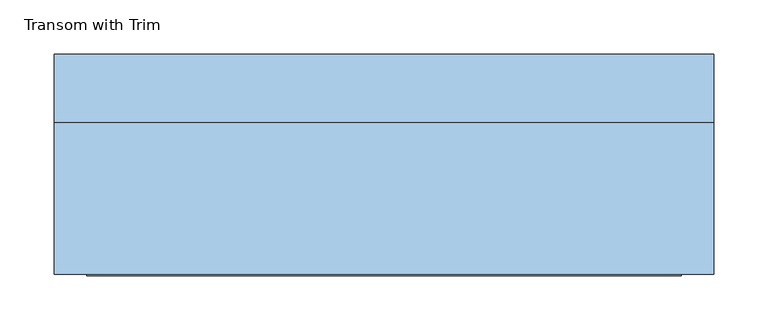
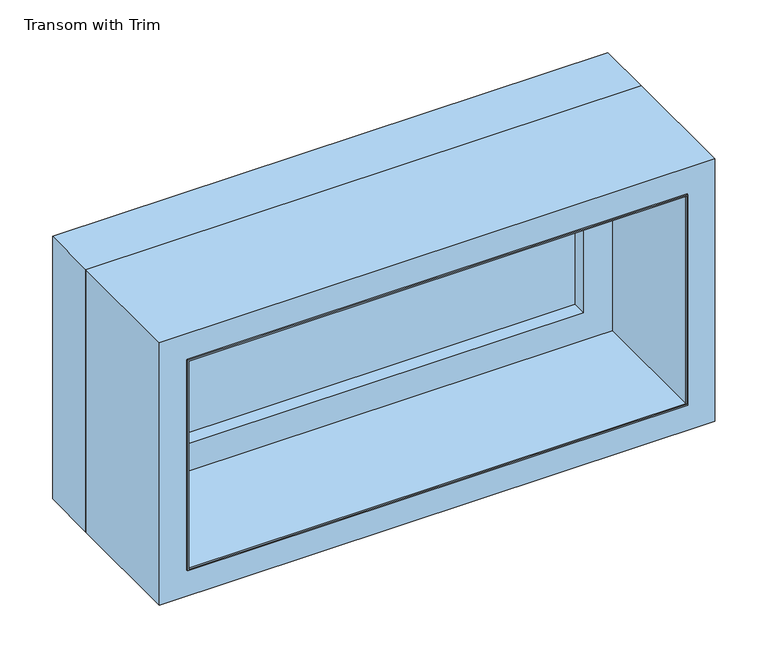
"""IFC4 building model written with IfcOpenShell, lengths in millimetres: window geometry, Transom with Trim : Haynes Transom."""

import ifcopenshell
import ifcopenshell.guid

model = None  # the IFC model being written
_history = None  # IfcOwnerHistory: only IFC2X3 demands one
_inside = {}  # id of a spatial element -> (the spatial element, [elements in it])
_under = {}  # id of a project, library or spatial element -> (it, [spatial elements below it])
_declared = {}  # id of a project -> (the project, [libraries it declares])
_typed = {}  # id of a type object -> (the type object, [elements of that type])
_made_of = {}  # id of a material, layer set ... -> (it, [elements and type objects made of it])


def new_model(schema):
    """Start an empty IFC model of exactly this schema.

    Asked for "IFC4X3", IfcOpenShell would pick the latest addendum, in which some entities
    have other attributes; the version numbers below select the first issue.
    IFC2X3 requires an IfcOwnerHistory on every rooted entity: one is made here for all.
    """
    global model, _history
    if schema == "IFC4X3":
        model = ifcopenshell.file(schema_version=(4, 3, 0, 0))
    else:
        model = ifcopenshell.file(schema=schema)
    _inside.clear()
    _under.clear()
    _declared.clear()
    _typed.clear()
    _made_of.clear()
    _history = None
    if model.schema == "IFC2X3":
        org = make("IfcOrganization", Name="unknown")
        user = make(
            "IfcPersonAndOrganization",
            ThePerson=make("IfcPerson", FamilyName="unknown"),
            TheOrganization=org,
        )
        app = make(
            "IfcApplication",
            ApplicationDeveloper=org,
            Version="unknown",
            ApplicationFullName="unknown",
            ApplicationIdentifier="unknown",
        )
        _history = make(
            "IfcOwnerHistory",
            OwningUser=user,
            OwningApplication=app,
            ChangeAction="ADDED",
            CreationDate=0,
        )
    return model


def make(cls, **values):
    """One entity of the class cls with the attributes given. An attribute that is None is left unset."""
    return model.create_entity(
        cls, **{name: value for name, value in values.items() if value is not None}
    )


def rooted(cls, **values):
    """An entity with a GlobalId (a new one), such as an element, a storey or a relation."""
    return make(cls, GlobalId=ifcopenshell.guid.new(), OwnerHistory=_history, **values)


def si_unit(unit_type, name, prefix=None):
    """IfcSIUnit, for example si_unit("LENGTHUNIT", "METRE", prefix="MILLI")."""
    return make("IfcSIUnit", UnitType=unit_type, Prefix=prefix, Name=name)


def assignment(units):
    """IfcUnitAssignment: the units of a project."""
    return None if units is None else make("IfcUnitAssignment", Units=units)


def point(xyz):
    """IfcCartesianPoint."""
    return None if xyz is None else make("IfcCartesianPoint", Coordinates=xyz)


def direction(xyz):
    """IfcDirection."""
    return None if xyz is None else make("IfcDirection", DirectionRatios=xyz)


def frame(location, z_axis=None, x_axis=None):
    """IfcAxis2Placement3D, a coordinate frame: its origin and axes. An axis left out is left unset."""
    return make(
        "IfcAxis2Placement3D",
        Location=point(location),
        Axis=direction(z_axis),
        RefDirection=direction(x_axis),
    )


def origin():
    """The frame at (0, 0, 0) with its axes left unset."""
    return frame((0.0, 0.0, 0.0))


def place(relative_to, where):
    """IfcLocalPlacement: puts the frame where relative to a parent placement (None: the world)."""
    return make(
        "IfcLocalPlacement", PlacementRelTo=relative_to, RelativePlacement=where
    )


def context(
    kind, dimensions, precision=None, world=None, true_north=None, identifier=None
):
    """IfcGeometricRepresentationContext, for example the 3D "Model" context."""
    return make(
        "IfcGeometricRepresentationContext",
        ContextIdentifier=identifier,
        ContextType=kind,
        CoordinateSpaceDimension=dimensions,
        Precision=precision,
        WorldCoordinateSystem=world,
        TrueNorth=true_north,
    )


def project(units=None, contexts=None):
    """IfcProject with its units and contexts."""
    return rooted(
        "IfcProject",
        Name="project",
        RepresentationContexts=contexts,
        UnitsInContext=assignment(units),
    )


def spatial(cls, under=None, at=None, **own):
    """A site, building, storey or space (cls), placed at a placement, below another one or the project."""
    s = rooted(cls, ObjectPlacement=at, **own)
    if under is not None:
        _under.setdefault(under.id(), (under, []))[1].append(s)
    return s


def polyline(points):
    """IfcPolyline through the points."""
    return make("IfcPolyline", Points=[point(p) for p in points])


def outline(outer, holes=None, kind="AREA"):
    """IfcArbitraryClosedProfileDef: a profile drawn as a closed curve; with holes, ...WithVoids."""
    if holes is None:
        return make("IfcArbitraryClosedProfileDef", ProfileType=kind, OuterCurve=outer)
    return make(
        "IfcArbitraryProfileDefWithVoids",
        ProfileType=kind,
        OuterCurve=outer,
        InnerCurves=holes,
    )


def extrude(swept, where, along, depth):
    """IfcExtrudedAreaSolid: the profile swept, set in the frame where, extruded along a direction by depth."""
    return make(
        "IfcExtrudedAreaSolid",
        SweptArea=swept,
        Position=where,
        ExtrudedDirection=direction(along),
        Depth=depth,
    )


def shape(context_of_items, identifier, shape_type, items):
    """IfcShapeRepresentation: the items that make up one representation, for example the "Body"."""
    return make(
        "IfcShapeRepresentation",
        ContextOfItems=context_of_items,
        RepresentationIdentifier=identifier,
        RepresentationType=shape_type,
        Items=items,
    )


def source(mapping_origin, context_of_items, identifier, shape_type, items):
    """IfcRepresentationMap: a shape defined once, which mapped items show again and again."""
    return make(
        "IfcRepresentationMap",
        MappingOrigin=mapping_origin,
        MappedRepresentation=shape(context_of_items, identifier, shape_type, items),
    )


def transform(
    local_origin,
    x_axis=None,
    y_axis=None,
    z_axis=None,
    scale=None,
    scale2=None,
    scale3=None,
    uniform=True,
):
    """IfcCartesianTransformationOperator3D, or its non-uniform kind. x_axis, y_axis, z_axis: its Axis1, 2, 3."""
    if uniform:
        return make(
            "IfcCartesianTransformationOperator3D",
            Axis1=direction(x_axis),
            Axis2=direction(y_axis),
            LocalOrigin=point(local_origin),
            Scale=scale,
            Axis3=direction(z_axis),
        )
    return make(
        "IfcCartesianTransformationOperator3DnonUniform",
        Axis1=direction(x_axis),
        Axis2=direction(y_axis),
        LocalOrigin=point(local_origin),
        Scale=scale,
        Axis3=direction(z_axis),
        Scale2=scale2,
        Scale3=scale3,
    )


def mapped(mapping_source, mapping_target):
    """IfcMappedItem: shows the shape of a source again, moved by a transform."""
    return make(
        "IfcMappedItem", MappingSource=mapping_source, MappingTarget=mapping_target
    )


def made_of(thing, what):
    """Note that an element or type object is made of a material, layer set ...; save() writes the relation."""
    if what is not None:
        _made_of.setdefault(what.id(), (what, []))[1].append(thing)
    return thing


def element(
    cls,
    number,
    at=None,
    inside=None,
    cuts=None,
    type_object=None,
    material=None,
    context=None,
    identifier="Body",
    shape_type=None,
    held_by="IfcProductDefinitionShape",
    body=None,
    shapes=None,
    **own,
):
    """One element of the class cls, such as IfcWall. Its Tag is "e" and its number.

    at: its placement. inside: the storey or other place that contains it. cuts: it is an
    opening in that element (IfcRelVoidsElement). A single representation is given by context,
    identifier, shape_type and body (its items); several are given by shapes. held_by: the class
    of the entity that holds the representations. save() writes the other relations.
    """
    e = rooted(cls, Tag="e%d" % number, ObjectPlacement=at, **own)
    if body is not None:
        shapes = [shape(context, identifier, shape_type, body)]
    if shapes is not None:
        e.Representation = make(held_by, Representations=shapes)
    if inside is not None:
        _inside.setdefault(inside.id(), (inside, []))[1].append(e)
    if cuts is not None:
        rooted(
            "IfcRelVoidsElement", RelatingBuildingElement=cuts, RelatedOpeningElement=e
        )
    if type_object is not None:
        _typed.setdefault(type_object.id(), (type_object, []))[1].append(e)
    return made_of(e, material)


def aggregate(whole, parts):
    """IfcRelAggregates: a whole, such as a stair, and the parts it consists of."""
    return rooted("IfcRelAggregates", RelatingObject=whole, RelatedObjects=parts)


def save(model, path):
    """Write the relations noted so far, then the file.

    IfcRelAggregates (storeys below a building ...), IfcRelContainedInSpatialStructure (elements
    in a storey), IfcRelDefinesByType, IfcRelAssociatesMaterial and IfcRelDeclares: one each for
    every whole, place, type object, material and project.
    """
    for whole, parts in _under.values():
        aggregate(whole, parts)
    for where, things in _inside.values():
        rooted(
            "IfcRelContainedInSpatialStructure",
            RelatedElements=things,
            RelatingStructure=where,
        )
    for kind, things in _typed.values():
        rooted("IfcRelDefinesByType", RelatedObjects=things, RelatingType=kind)
    for what, things in _made_of.values():
        rooted("IfcRelAssociatesMaterial", RelatedObjects=things, RelatingMaterial=what)
    for by, libraries in _declared.values():
        rooted("IfcRelDeclares", RelatingContext=by, RelatedDefinitions=libraries)
    model.write(path)


def transom_with_trim_e78fe0c8(model_context):
    return source(origin(), model_context, "Body", "SweptSolid", [
        extrude(outline(polyline([(2103.4375, 236.5375), (2103.4375, -312.7375), (1858.9625, -312.7375), (1858.9625, 236.5375), (2103.4375, 236.5375)]), holes=[polyline([(2101.85, 234.95), (1860.55, 234.95), (1860.55, -311.15), (2101.85, -311.15), (2101.85, 234.95)])]), frame((0.0, -103.1875, 0.0), z_axis=(0.0, 1.0, 0.0), x_axis=(0.0, 0.0, 1.0)), (0.0, 0.0, 1.0), 1.5875),
        extrude(outline(polyline([(203.2, 53.975), (-279.4, 53.975), (-279.4, 66.675), (203.2, 66.675), (203.2, 53.975)])), frame((0.0, 0.0, 1892.3), z_axis=(0.0, 0.0, 1.0), x_axis=(1.0, 0.0, 0.0)), (0.0, 0.0, 1.0), 177.8),
        extrude(outline(polyline([(2114.55, -323.85), (1847.85, -323.85), (1847.85, 247.65), (2114.55, 247.65), (2114.55, -323.85)]), holes=[polyline([(2070.1, -279.4), (2070.1, 203.2), (1892.3, 203.2), (1892.3, -279.4), (2070.1, -279.4)])]), frame((0.0, 38.1, 0.0), z_axis=(0.0, 1.0, 0.0), x_axis=(0.0, 0.0, 1.0)), (0.0, 0.0, 1.0), 44.45),
        extrude(outline(polyline([(2133.6, -342.9), (1828.8, -342.9), (1828.8, 266.7), (2133.6, 266.7), (2133.6, -342.9)]), holes=[polyline([(2101.85, -311.15), (2101.85, 234.95), (1860.55, 234.95), (1860.55, -311.15), (2101.85, -311.15)])]), frame((0.0, -101.6, 0.0), z_axis=(0.0, 1.0, 0.0), x_axis=(0.0, 0.0, 1.0)), (0.0, 0.0, 1.0), 139.7),
        extrude(outline(polyline([(2133.6, 266.7), (2133.6, -342.9), (1828.8, -342.9), (1828.8, 266.7), (2133.6, 266.7)]), holes=[polyline([(2114.55, 247.65), (1847.85, 247.65), (1847.85, -323.85), (2114.55, -323.85), (2114.55, 247.65)])]), frame((0.0, 38.1, 0.0), z_axis=(0.0, 1.0, 0.0), x_axis=(0.0, 0.0, 1.0)), (0.0, 0.0, 1.0), 63.5),
    ])


if __name__ == "__main__":
    model = new_model("IFC4")
    model_context = context("Model", 3, world=origin())
    ifc_project = project(units=[si_unit("LENGTHUNIT", "METRE", prefix="MILLI")], contexts=[model_context])
    site = spatial("IfcSite", under=ifc_project)
    building = spatial("IfcBuilding", under=site)
    placement = place(None, origin())
    transom_with_trim_shape = transom_with_trim_e78fe0c8(model_context)
    element("IfcWindow", 1, ObjectType="Transom with Trim : Haynes Transom", at=placement, inside=building, context=model_context, shape_type="MappedRepresentation", body=[
        mapped(transom_with_trim_shape, transform((0.0, 0.0, 0.0), x_axis=(1.0, 0.0, 0.0), y_axis=(0.0, 1.0, 0.0), z_axis=(0.0, 0.0, 1.0))),
    ])
    save(model, "model.ifc")

# Revit data of these elements
# Type "Transom with Trim : Haynes Transom"
#   Type Mark = "30"
#   Assembly Code = "B2020100"
#   Height = 1' - 0"
#   Default Sill Height = 6' - 0"
#   Trim Projection - Ext. = 0' - 0 1/16"
#   Trim Projection - Int. = 0' - 0 1/16"
#   Trim Width - Exterior = 0' - 0 1/16"
#   Trim Width - Interior = 0' - 0 1/16"
#   Width = 2' - 0"
#   Window Inset = 0' - 0 3/4"
#   Glass Pane Material = Glass
#   Sash Material = Sash
#   Trim Exterior Material = Trim
#   Trim Interior Material = Trim
#   Wall Closure = (empty or 0)
# Element 1 (IfcWindow, "Transom with Trim : Haynes Transom")
#   Materials on its faces: "Sash", "Trim", "Glass"
# Materials
#   "Glass": class "Glass", colour RGB 0 128 192, transparency 0.75
#   "Sash": class "Wood", colour RGB 224 178 126, transparency 0
#   "Trim": class "Wood", colour RGB 224 178 126, transparency 0
